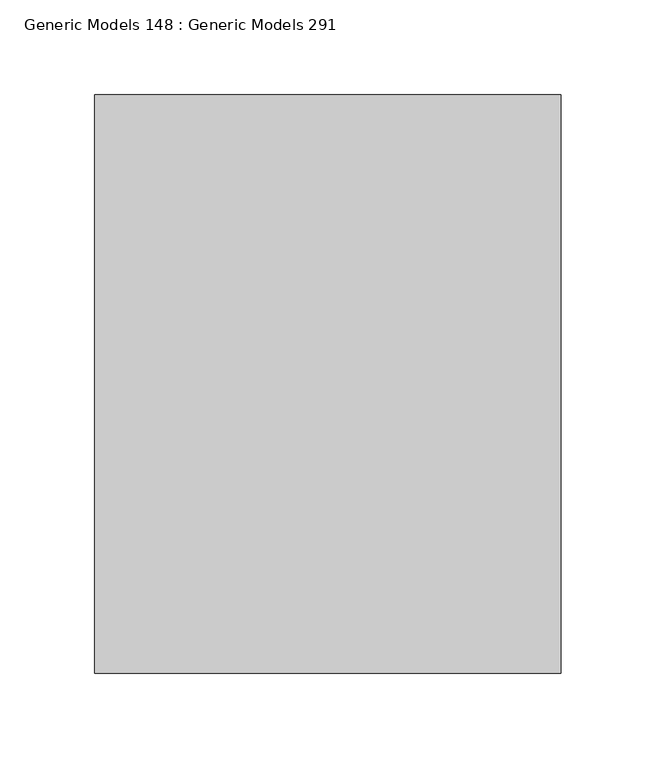
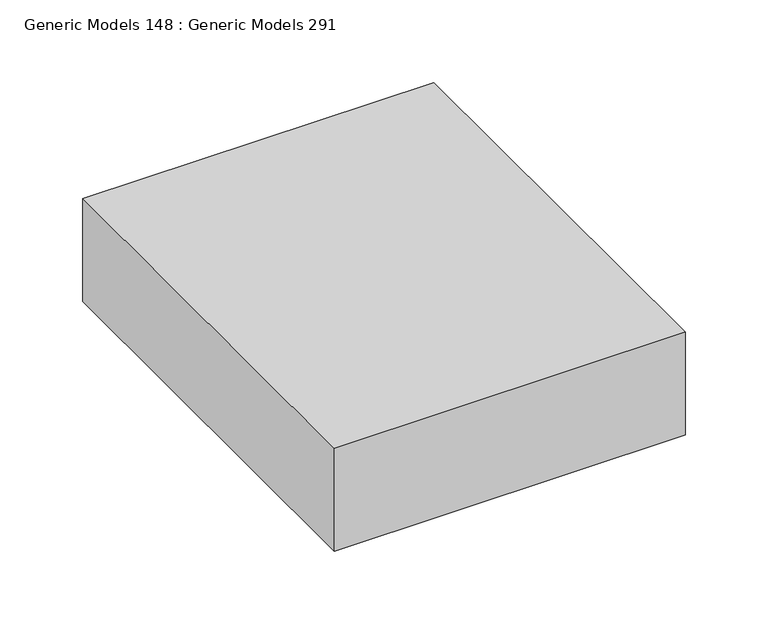
"""IFC4 building model written with IfcOpenShell, lengths in millimetres: proxy geometry, Generic Models 148 : Generic Models 291."""

from ifc_helpers import new_model, si_unit, frame, origin, place, context, project, spatial, polyline, outline, extrude, source, transform, mapped, element, save


def generic_models_148_generic_models_291_9717d98d(model_context):
    return source(origin(), model_context, "Body", "SweptSolid", [
        extrude(outline(polyline([(7129.008082, 8214.8672747), (6883.2263704, 8214.8672747), (6883.2263704, 8519.6672747), (7129.008082, 8519.6672747), (7129.008082, 8214.8672747)])), frame((0.0, 0.0, 123297.696), z_axis=(0.0, 0.0, 1.0), x_axis=(1.0, 0.0, 0.0)), (0.0, 0.0, 1.0), 76.2),
    ])


if __name__ == "__main__":
    model = new_model("IFC4")
    model_context = context("Model", 3, world=origin())
    ifc_project = project(units=[si_unit("LENGTHUNIT", "METRE", prefix="MILLI")], contexts=[model_context])
    site = spatial("IfcSite", under=ifc_project)
    building = spatial("IfcBuilding", under=site)
    placement = place(None, origin())
    generic_models_148_generic_models_291_shape = generic_models_148_generic_models_291_9717d98d(model_context)
    element("IfcBuildingElementProxy", 1, Name="Generic Models 148 : Generic Models 291", ObjectType="Generic Models 148 : Generic Models 291", at=placement, inside=building, context=model_context, shape_type="MappedRepresentation", body=[
        mapped(generic_models_148_generic_models_291_shape, transform((0.0, 0.0, 0.0), x_axis=(1.0, 0.0, 0.0), y_axis=(0.0, 1.0, 0.0), z_axis=(0.0, 0.0, 1.0))),
    ])
    save(model, "model.ifc")

# Revit data of these elements
# Element 1 (IfcBuildingElementProxy, "Generic Models 148 : Generic Models 291")
#   Materials on its faces: "_LANDSCAPING STONE T.B.D."
# Materials
#   "_LANDSCAPING STONE T.B.D.": class "Generic", colour RGB 122 131 148, transparency 0, Cost = 0
